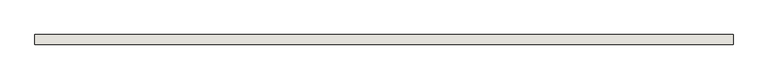
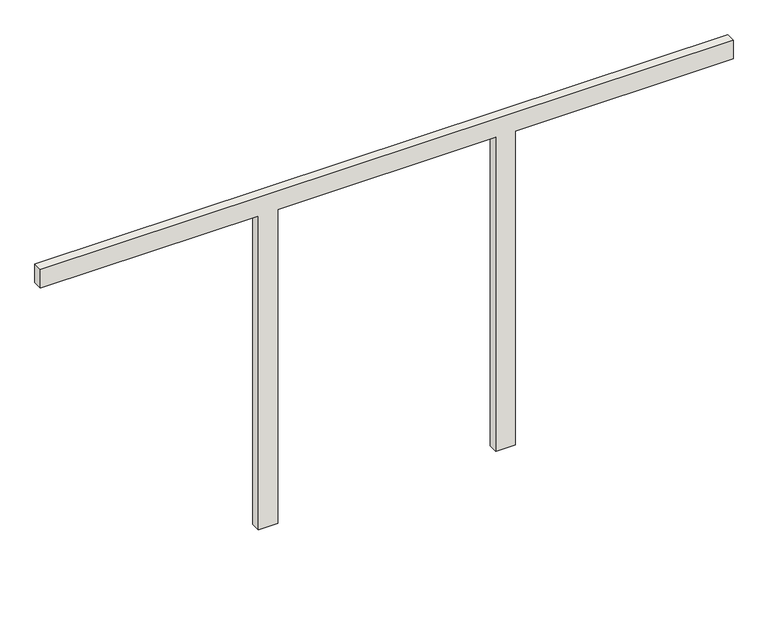
"""IFC4 building model written with IfcOpenShell, lengths in millimetres: wall geometry, 0_3d."""

from ifc_helpers import new_model, si_unit, frame, origin, place, context, project, spatial, polyline, outline, extrude, source, transform, mapped, element, save


def wall_37c49f1e(model_context):
    return source(origin(), model_context, "Body", "SweptSolid", [
        extrude(outline(polyline([(0.0, 3886.7), (2720.0, 3886.7), (2720.0, 5670.0), (2880.0, 5670.0), (2880.0, 0.0), (2720.0, 0.0), (2720.0, 1783.4), (0.0, 1783.4), (0.0, 1943.4), (2720.0, 1943.4), (2720.0, 3726.7), (0.0, 3726.7), (0.0, 3886.7)])), frame((0.0, 0.0, 0.0), z_axis=(0.0, 1.0, 0.0), x_axis=(0.0, 0.0, 1.0)), (0.0, 0.0, 1.0), 78.0),
    ])


if __name__ == "__main__":
    model = new_model("IFC4")
    model_context = context("Model", 3, world=origin())
    ifc_project = project(units=[si_unit("LENGTHUNIT", "METRE", prefix="MILLI")], contexts=[model_context])
    site = spatial("IfcSite", under=ifc_project)
    building = spatial("IfcBuilding", under=site)
    placement = place(None, origin())
    wall_shape = wall_37c49f1e(model_context)
    element("IfcWall", 1, ObjectType="0_3d", at=placement, inside=building, context=model_context, shape_type="MappedRepresentation", body=[
        mapped(wall_shape, transform((0.0, 0.0, 0.0), x_axis=(1.0, 0.0, 0.0), y_axis=(0.0, 1.0, 0.0), z_axis=(0.0, 0.0, 1.0))),
    ])
    save(model, "model.ifc")

# Revit data of these elements
# Element 1 (IfcWall, "0_3d")
#   Materials on its faces: "glas"
# Materials
#   "glas": class "Unassigned", colour RGB 250 253 254, transparency 0.95
